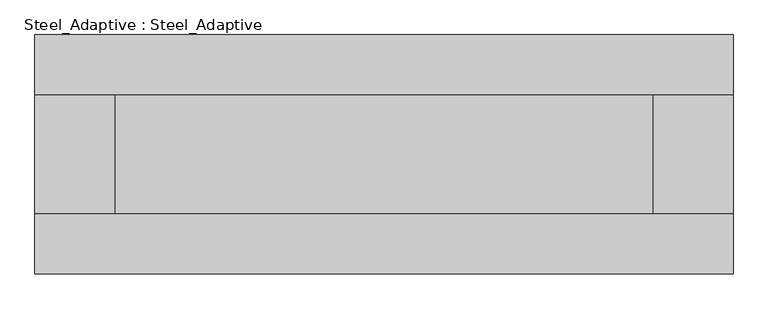
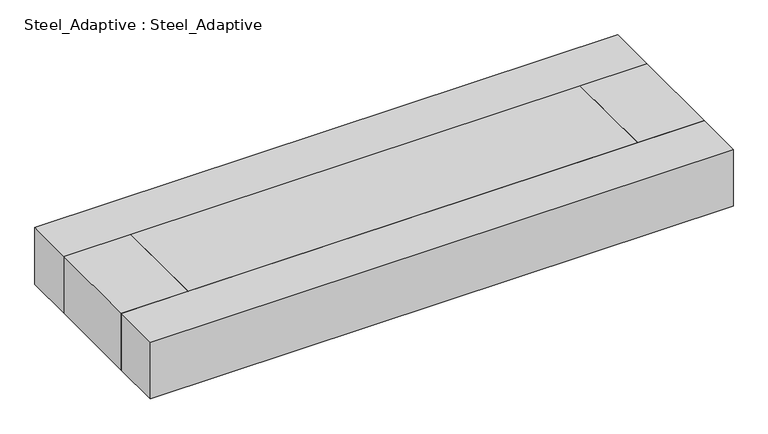
"""IFC4 building model written with IfcOpenShell, lengths in millimetres: proxy geometry, Steel_Adaptive : Steel_Adaptive."""

from ifc_helpers import new_model, si_unit, frame, origin, place, context, project, spatial, polyline, outline, extrude, source, transform, mapped, element, save


def steel_adaptive_steel_adaptive_eb98373c(model_context):
    return source(origin(), model_context, "Body", "SweptSolid", [
        extrude(outline(polyline([(8750.0, 1500.0), (-8750.0, 1500.0), (-8750.0, 3000.0), (8750.0, 3000.0), (8750.0, 1500.0)])), frame((0.0, 0.0, 104400.0), z_axis=(0.0, 0.0, 1.0), x_axis=(1.0, 0.0, 0.0)), (0.0, 0.0, 1.0), 1800.0),
        extrude(outline(polyline([(-8750.0, -1500.0), (8750.0, -1500.0), (8750.0, -3000.0), (-8750.0, -3000.0), (-8750.0, -1500.0)])), frame((0.0, 0.0, 104400.0), z_axis=(0.0, 0.0, 1.0), x_axis=(1.0, 0.0, 0.0)), (0.0, 0.0, 1.0), 1800.0),
        extrude(outline(polyline([(6750.0, -1500.0), (6750.0, 1500.0), (8750.0, 1500.0), (8750.0, -1500.0), (6750.0, -1500.0)])), frame((0.0, 0.0, 104400.0), z_axis=(0.0, 0.0, 1.0), x_axis=(1.0, 0.0, 0.0)), (0.0, 0.0, 1.0), 1800.0),
        extrude(outline(polyline([(-6750.0, 1500.0), (-6750.0, -1500.0), (-8750.0, -1500.0), (-8750.0, 1500.0), (-6750.0, 1500.0)])), frame((0.0, 0.0, 104400.0), z_axis=(0.0, 0.0, 1.0), x_axis=(1.0, 0.0, 0.0)), (0.0, 0.0, 1.0), 1800.0),
        extrude(outline(polyline([(-6750.0, -1500.0), (-6750.0, 1500.0), (6750.0, 1500.0), (6750.0, -1500.0), (-6750.0, -1500.0)])), frame((0.0, 0.0, 104400.0), z_axis=(0.0, 0.0, 1.0), x_axis=(1.0, 0.0, 0.0)), (0.0, 0.0, 1.0), 1800.0),
    ])


if __name__ == "__main__":
    model = new_model("IFC4")
    model_context = context("Model", 3, world=origin())
    ifc_project = project(units=[si_unit("LENGTHUNIT", "METRE", prefix="MILLI")], contexts=[model_context])
    site = spatial("IfcSite", under=ifc_project)
    building = spatial("IfcBuilding", under=site)
    placement = place(None, origin())
    steel_adaptive_steel_adaptive_shape = steel_adaptive_steel_adaptive_eb98373c(model_context)
    element("IfcBuildingElementProxy", 1, Name="Steel_Adaptive : Steel_Adaptive", ObjectType="Steel_Adaptive : Steel_Adaptive", at=placement, inside=building, context=model_context, shape_type="MappedRepresentation", body=[
        mapped(steel_adaptive_steel_adaptive_shape, transform((0.0, 0.0, 0.0), x_axis=(1.0, 0.0, 0.0), y_axis=(0.0, 1.0, 0.0), z_axis=(0.0, 0.0, 1.0))),
    ])
    save(model, "model.ifc")

# Revit data of these elements
# Type "Steel_Adaptive : Steel_Adaptive"
#   Width = 3000 mm
#   Top Width = 3000 mm
#   Length = 21000 mm
#   Height [instance default] = 80000 mm
#   Default Elevation = 0
# Element 1 (IfcBuildingElementProxy, "Steel_Adaptive : Steel_Adaptive")
#   Height = 104400 mm
